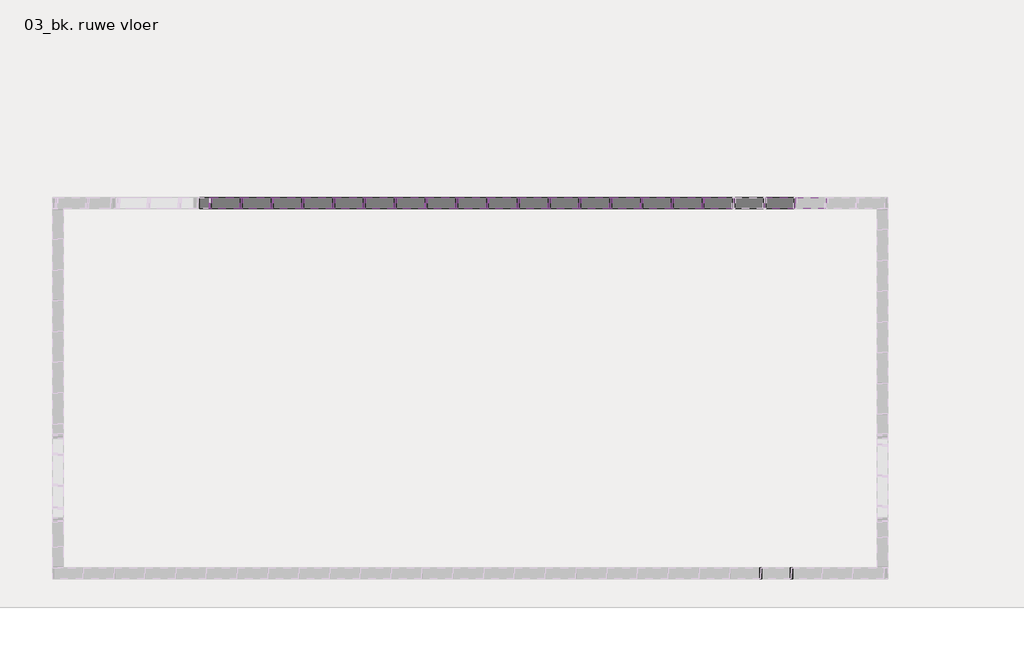
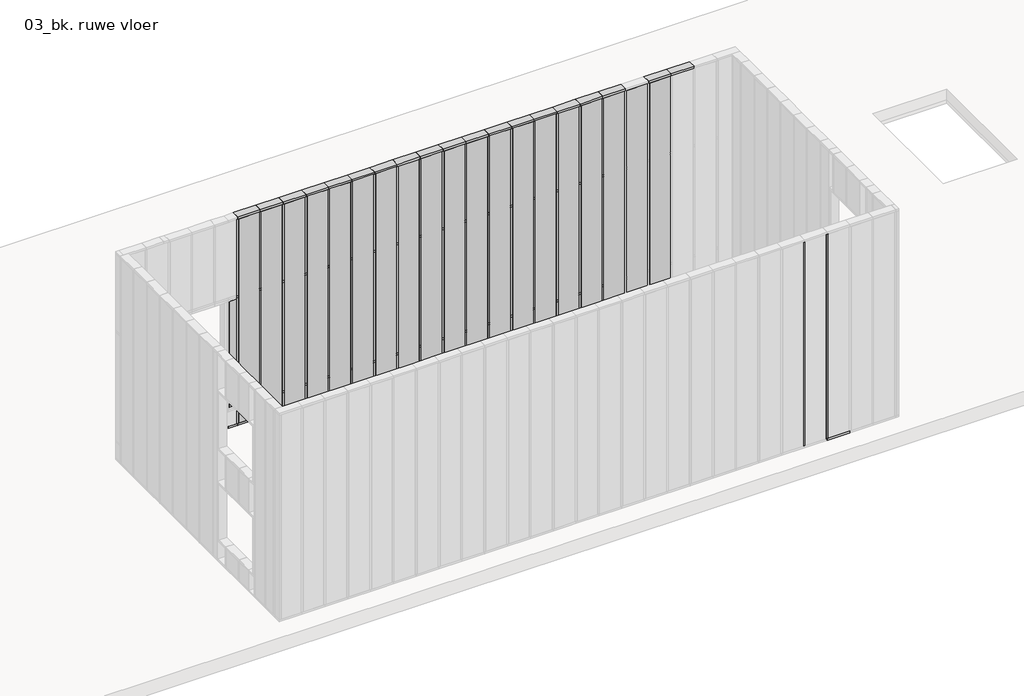
# One storey, part 3 of 9: 124 members, 20 plates.
"""IFC4 building model written with IfcOpenShell, lengths in millimetres."""

import ifcopenshell
import ifcopenshell.guid

model = None  # the IFC model being written
_history = None  # IfcOwnerHistory: only IFC2X3 demands one
_inside = {}  # id of a spatial element -> (the spatial element, [elements in it])
_under = {}  # id of a project, library or spatial element -> (it, [spatial elements below it])
_declared = {}  # id of a project -> (the project, [libraries it declares])
_typed = {}  # id of a type object -> (the type object, [elements of that type])
_made_of = {}  # id of a material, layer set ... -> (it, [elements and type objects made of it])


def new_model(schema):
    """Start an empty IFC model of exactly this schema.

    Asked for "IFC4X3", IfcOpenShell would pick the latest addendum, in which some entities
    have other attributes; the version numbers below select the first issue.
    IFC2X3 requires an IfcOwnerHistory on every rooted entity: one is made here for all.
    """
    global model, _history
    if schema == "IFC4X3":
        model = ifcopenshell.file(schema_version=(4, 3, 0, 0))
    else:
        model = ifcopenshell.file(schema=schema)
    _inside.clear()
    _under.clear()
    _declared.clear()
    _typed.clear()
    _made_of.clear()
    _history = None
    if model.schema == "IFC2X3":
        org = make("IfcOrganization", Name="unknown")
        user = make(
            "IfcPersonAndOrganization",
            ThePerson=make("IfcPerson", FamilyName="unknown"),
            TheOrganization=org,
        )
        app = make(
            "IfcApplication",
            ApplicationDeveloper=org,
            Version="unknown",
            ApplicationFullName="unknown",
            ApplicationIdentifier="unknown",
        )
        _history = make(
            "IfcOwnerHistory",
            OwningUser=user,
            OwningApplication=app,
            ChangeAction="ADDED",
            CreationDate=0,
        )
    return model


def make(cls, **values):
    """One entity of the class cls with the attributes given. An attribute that is None is left unset."""
    return model.create_entity(
        cls, **{name: value for name, value in values.items() if value is not None}
    )


def rooted(cls, **values):
    """An entity with a GlobalId (a new one), such as an element, a storey or a relation."""
    return make(cls, GlobalId=ifcopenshell.guid.new(), OwnerHistory=_history, **values)


def si_unit(unit_type, name, prefix=None):
    """IfcSIUnit, for example si_unit("LENGTHUNIT", "METRE", prefix="MILLI")."""
    return make("IfcSIUnit", UnitType=unit_type, Prefix=prefix, Name=name)


def assignment(units):
    """IfcUnitAssignment: the units of a project."""
    return None if units is None else make("IfcUnitAssignment", Units=units)


def point(xyz):
    """IfcCartesianPoint."""
    return None if xyz is None else make("IfcCartesianPoint", Coordinates=xyz)


def direction(xyz):
    """IfcDirection."""
    return None if xyz is None else make("IfcDirection", DirectionRatios=xyz)


def frame(location, z_axis=None, x_axis=None):
    """IfcAxis2Placement3D, a coordinate frame: its origin and axes. An axis left out is left unset."""
    return make(
        "IfcAxis2Placement3D",
        Location=point(location),
        Axis=direction(z_axis),
        RefDirection=direction(x_axis),
    )


def origin():
    """The frame at (0, 0, 0) with its axes left unset."""
    return frame((0.0, 0.0, 0.0))


def origin_with_axes():
    """The frame at (0, 0, 0) with the z axis (0, 0, 1) and the x axis (1, 0, 0) written out."""
    return frame((0.0, 0.0, 0.0), z_axis=(0.0, 0.0, 1.0), x_axis=(1.0, 0.0, 0.0))


def place(relative_to, where):
    """IfcLocalPlacement: puts the frame where relative to a parent placement (None: the world)."""
    return make(
        "IfcLocalPlacement", PlacementRelTo=relative_to, RelativePlacement=where
    )


def context(
    kind, dimensions, precision=None, world=None, true_north=None, identifier=None
):
    """IfcGeometricRepresentationContext, for example the 3D "Model" context."""
    return make(
        "IfcGeometricRepresentationContext",
        ContextIdentifier=identifier,
        ContextType=kind,
        CoordinateSpaceDimension=dimensions,
        Precision=precision,
        WorldCoordinateSystem=world,
        TrueNorth=true_north,
    )


def project(units=None, contexts=None):
    """IfcProject with its units and contexts."""
    return rooted(
        "IfcProject",
        Name="project",
        RepresentationContexts=contexts,
        UnitsInContext=assignment(units),
    )


def spatial(cls, under=None, at=None, **own):
    """A site, building, storey or space (cls), placed at a placement, below another one or the project."""
    s = rooted(cls, ObjectPlacement=at, **own)
    if under is not None:
        _under.setdefault(under.id(), (under, []))[1].append(s)
    return s


def polyline(points):
    """IfcPolyline through the points."""
    return make("IfcPolyline", Points=[point(p) for p in points])


def outline(outer, holes=None, kind="AREA"):
    """IfcArbitraryClosedProfileDef: a profile drawn as a closed curve; with holes, ...WithVoids."""
    if holes is None:
        return make("IfcArbitraryClosedProfileDef", ProfileType=kind, OuterCurve=outer)
    return make(
        "IfcArbitraryProfileDefWithVoids",
        ProfileType=kind,
        OuterCurve=outer,
        InnerCurves=holes,
    )


def extrude(swept, where, along, depth):
    """IfcExtrudedAreaSolid: the profile swept, set in the frame where, extruded along a direction by depth."""
    return make(
        "IfcExtrudedAreaSolid",
        SweptArea=swept,
        Position=where,
        ExtrudedDirection=direction(along),
        Depth=depth,
    )


def shape(context_of_items, identifier, shape_type, items):
    """IfcShapeRepresentation: the items that make up one representation, for example the "Body"."""
    return make(
        "IfcShapeRepresentation",
        ContextOfItems=context_of_items,
        RepresentationIdentifier=identifier,
        RepresentationType=shape_type,
        Items=items,
    )


def source(mapping_origin, context_of_items, identifier, shape_type, items):
    """IfcRepresentationMap: a shape defined once, which mapped items show again and again."""
    return make(
        "IfcRepresentationMap",
        MappingOrigin=mapping_origin,
        MappedRepresentation=shape(context_of_items, identifier, shape_type, items),
    )


def transform(
    local_origin,
    x_axis=None,
    y_axis=None,
    z_axis=None,
    scale=None,
    scale2=None,
    scale3=None,
    uniform=True,
):
    """IfcCartesianTransformationOperator3D, or its non-uniform kind. x_axis, y_axis, z_axis: its Axis1, 2, 3."""
    if uniform:
        return make(
            "IfcCartesianTransformationOperator3D",
            Axis1=direction(x_axis),
            Axis2=direction(y_axis),
            LocalOrigin=point(local_origin),
            Scale=scale,
            Axis3=direction(z_axis),
        )
    return make(
        "IfcCartesianTransformationOperator3DnonUniform",
        Axis1=direction(x_axis),
        Axis2=direction(y_axis),
        LocalOrigin=point(local_origin),
        Scale=scale,
        Axis3=direction(z_axis),
        Scale2=scale2,
        Scale3=scale3,
    )


def mapped(mapping_source, mapping_target):
    """IfcMappedItem: shows the shape of a source again, moved by a transform."""
    return make(
        "IfcMappedItem", MappingSource=mapping_source, MappingTarget=mapping_target
    )


def made_of(thing, what):
    """Note that an element or type object is made of a material, layer set ...; save() writes the relation."""
    if what is not None:
        _made_of.setdefault(what.id(), (what, []))[1].append(thing)
    return thing


def element(
    cls,
    number,
    at=None,
    inside=None,
    cuts=None,
    type_object=None,
    material=None,
    context=None,
    identifier="Body",
    shape_type=None,
    held_by="IfcProductDefinitionShape",
    body=None,
    shapes=None,
    **own,
):
    """One element of the class cls, such as IfcWall. Its Tag is "e" and its number.

    at: its placement. inside: the storey or other place that contains it. cuts: it is an
    opening in that element (IfcRelVoidsElement). A single representation is given by context,
    identifier, shape_type and body (its items); several are given by shapes. held_by: the class
    of the entity that holds the representations. save() writes the other relations.
    """
    e = rooted(cls, Tag="e%d" % number, ObjectPlacement=at, **own)
    if body is not None:
        shapes = [shape(context, identifier, shape_type, body)]
    if shapes is not None:
        e.Representation = make(held_by, Representations=shapes)
    if inside is not None:
        _inside.setdefault(inside.id(), (inside, []))[1].append(e)
    if cuts is not None:
        rooted(
            "IfcRelVoidsElement", RelatingBuildingElement=cuts, RelatedOpeningElement=e
        )
    if type_object is not None:
        _typed.setdefault(type_object.id(), (type_object, []))[1].append(e)
    return made_of(e, material)


def aggregate(whole, parts):
    """IfcRelAggregates: a whole, such as a stair, and the parts it consists of."""
    return rooted("IfcRelAggregates", RelatingObject=whole, RelatedObjects=parts)


def save(model, path):
    """Write the relations noted so far, then the file.

    IfcRelAggregates (storeys below a building ...), IfcRelContainedInSpatialStructure (elements
    in a storey), IfcRelDefinesByType, IfcRelAssociatesMaterial and IfcRelDeclares: one each for
    every whole, place, type object, material and project.
    """
    for whole, parts in _under.values():
        aggregate(whole, parts)
    for where, things in _inside.values():
        rooted(
            "IfcRelContainedInSpatialStructure",
            RelatedElements=things,
            RelatingStructure=where,
        )
    for kind, things in _typed.values():
        rooted("IfcRelDefinesByType", RelatedObjects=things, RelatingType=kind)
    for what, things in _made_of.values():
        rooted("IfcRelAssociatesMaterial", RelatedObjects=things, RelatingMaterial=what)
    for by, libraries in _declared.values():
        rooted("IfcRelDeclares", RelatingContext=by, RelatedDefinitions=libraries)
    model.write(path)


def rectangular_mullion_51268c3e(model_context):
    return source(origin(), model_context, "Body", "SweptSolid", [
        extrude(outline(polyline([(0.0, -71.0), (-38.0, -71.0), (-38.0, 71.0), (0.0, 71.0), (0.0, -71.0)])), frame((0.0, 0.0, -407.0), z_axis=(0.0, 0.0, 1.0), x_axis=(1.0, 0.0, 0.0)), (0.0, 0.0, 1.0), 407.0),
    ])


def rectangular_mullion_fd8aedfe(model_context):
    return source(origin(), model_context, "Body", "SweptSolid", [
        extrude(outline(polyline([(-38.0, -71.0), (-38.0, 71.0), (0.0, 71.0), (0.0, -71.0), (-38.0, -71.0)])), frame((0.0, 0.0, -407.0), z_axis=(0.0, 0.0, 1.0), x_axis=(1.0, 0.0, 0.0)), (0.0, 0.0, 1.0), 407.0),
    ])


def rectangular_mullion_bc699282(model_context):
    return source(origin(), model_context, "Body", "SweptSolid", [
        extrude(outline(polyline([(19.0, -71.0), (-19.0, -71.0), (-19.0, 71.0), (19.0, 71.0), (19.0, -71.0)])), frame((0.0, 0.0, -3849.0), z_axis=(0.0, 0.0, 1.0), x_axis=(1.0, 0.0, 0.0)), (0.0, 0.0, 1.0), 3849.0),
    ])


def rectangular_mullion_c53917db(model_context):
    return source(origin(), model_context, "Body", "SweptSolid", [
        extrude(outline(polyline([(19.0, -71.0), (-19.0, -71.0), (-19.0, 71.0), (19.0, 71.0), (19.0, -71.0)])), frame((0.0, 0.0, -295.0), z_axis=(0.0, 0.0, 1.0), x_axis=(1.0, 0.0, 0.0)), (0.0, 0.0, 1.0), 295.0),
    ])


def rectangular_mullion_c6f7c22d(model_context):
    return source(origin(), model_context, "Body", "SweptSolid", [
        extrude(outline(polyline([(-38.0, -71.0), (-38.0, 71.0), (0.0, 71.0), (0.0, -71.0), (-38.0, -71.0)])), frame((0.0, 0.0, -167.1558939), z_axis=(0.0, 0.0, 1.0), x_axis=(1.0, 0.0, 0.0)), (0.0, 0.0, 1.0), 167.1558939),
    ])


def rectangular_mullion_878a7b4c(model_context):
    return source(origin(), model_context, "Body", "SweptSolid", [
        extrude(outline(polyline([(19.0, -71.0), (-19.0, -71.0), (-19.0, 71.0), (19.0, 71.0), (19.0, -71.0)])), frame((0.0, 0.0, -1440.0), z_axis=(0.0, 0.0, 1.0), x_axis=(1.0, 0.0, 0.0)), (0.0, 0.0, 1.0), 1440.0),
    ])


def rectangular_mullion_c09c4bb1(model_context):
    return source(origin(), model_context, "Body", "SweptSolid", [
        extrude(outline(polyline([(19.0, -71.0), (-19.0, -71.0), (-19.0, 71.0), (19.0, 71.0), (19.0, -71.0)])), frame((0.0, 0.0, -38.0), z_axis=(0.0, 0.0, 1.0), x_axis=(1.0, 0.0, 0.0)), (0.0, 0.0, 1.0), 38.0),
    ])


def rectangular_mullion_39366410(model_context):
    return source(origin(), model_context, "Body", "SweptSolid", [
        extrude(outline(polyline([(19.0, -71.0), (-19.0, -71.0), (-19.0, 71.0), (19.0, 71.0), (19.0, -71.0)])), frame((0.0, 0.0, -2038.0), z_axis=(0.0, 0.0, 1.0), x_axis=(1.0, 0.0, 0.0)), (0.0, 0.0, 1.0), 2038.0),
    ])


def system_panel_efc5a8ab(model_context):
    return source(origin(), model_context, "Body", "SweptSolid", [
        extrude(outline(polyline([(0.0, -184.5), (0.0, 184.5), (295.0, 184.5), (333.0, 184.5), (2371.0, 184.5), (2409.0, 184.5), (3849.0, 184.5), (3849.0, -184.5), (2409.0, -184.5), (2371.0, -184.5), (333.0, -184.5), (295.0, -184.5), (0.0, -184.5)])), frame((0.0, -71.0, 0.0), z_axis=(0.0, 1.0, 0.0), x_axis=(0.0, 0.0, 1.0)), (0.0, 0.0, 1.0), 142.0),
    ])


def system_panel_6860f7c2(model_context):
    return source(origin(), model_context, "Body", "SweptSolid", [
        extrude(outline(polyline([(64.577947, -71.0), (-64.577947, -71.0), (-64.577947, 71.0), (64.577947, 71.0), (64.577947, -71.0)])), origin_with_axes(), (0.0, 0.0, 1.0), 2000.0),
    ])


model = new_model("IFC4")

# Units and contexts
model_context = context("Model", 3, world=origin())
ifc_project = project(units=[si_unit("LENGTHUNIT", "METRE", prefix="MILLI")], contexts=[model_context])

# Site, building, storey
site = spatial("IfcSite", under=ifc_project)
building = spatial("IfcBuilding", under=site)
storey = spatial("IfcBuildingStorey", under=building, Name="03_bk. ruwe vloer", Elevation=11330.0)

# Members
placement = place(None, origin())
rectangular_mullion_shape = rectangular_mullion_51268c3e(model_context)
element("IfcMember", 1, ObjectType="Rectangular Mullion", at=placement, inside=storey, context=model_context, shape_type="MappedRepresentation", body=[
    mapped(rectangular_mullion_shape, transform((63849.9999997, 5200.0, 15255.0), x_axis=(0.0, 0.0, 1.0), y_axis=(0.0, 1.0, 0.0), z_axis=(-1.0, 0.0, 0.0))),
])
element("IfcMember", 2, ObjectType="Rectangular Mullion", at=placement, inside=storey, context=model_context, shape_type="MappedRepresentation", body=[
    mapped(rectangular_mullion_shape, transform((63442.9999997, 5200.0, 15255.0), x_axis=(0.0, 0.0, 1.0), y_axis=(0.0, 1.0, 0.0), z_axis=(-1.0, 0.0, 0.0))),
])
element("IfcMember", 3, ObjectType="Rectangular Mullion", at=placement, inside=storey, context=model_context, shape_type="MappedRepresentation", body=[
    mapped(rectangular_mullion_shape, transform((62628.9999997, 5200.0, 15255.0), x_axis=(0.0, 0.0, 1.0), y_axis=(0.0, 1.0, 0.0), z_axis=(-1.0, 0.0, 0.0))),
])
element("IfcMember", 4, ObjectType="Rectangular Mullion", at=placement, inside=storey, context=model_context, shape_type="MappedRepresentation", body=[
    mapped(rectangular_mullion_shape, transform((62221.9999997, 5200.0, 15255.0), x_axis=(0.0, 0.0, 1.0), y_axis=(0.0, 1.0, 0.0), z_axis=(-1.0, 0.0, 0.0))),
])
element("IfcMember", 5, ObjectType="Rectangular Mullion", at=placement, inside=storey, context=model_context, shape_type="MappedRepresentation", body=[
    mapped(rectangular_mullion_shape, transform((61814.9999997, 5200.0, 15255.0), x_axis=(0.0, 0.0, 1.0), y_axis=(0.0, 1.0, 0.0), z_axis=(-1.0, 0.0, 0.0))),
])
element("IfcMember", 6, ObjectType="Rectangular Mullion", at=placement, inside=storey, context=model_context, shape_type="MappedRepresentation", body=[
    mapped(rectangular_mullion_shape, transform((61407.9999997, 5200.0, 15255.0), x_axis=(0.0, 0.0, 1.0), y_axis=(0.0, 1.0, 0.0), z_axis=(-1.0, 0.0, 0.0))),
])
element("IfcMember", 7, ObjectType="Rectangular Mullion", at=placement, inside=storey, context=model_context, shape_type="MappedRepresentation", body=[
    mapped(rectangular_mullion_shape, transform((61000.9999997, 5200.0, 15255.0), x_axis=(0.0, 0.0, 1.0), y_axis=(0.0, 1.0, 0.0), z_axis=(-1.0, 0.0, 0.0))),
])
element("IfcMember", 8, ObjectType="Rectangular Mullion", at=placement, inside=storey, context=model_context, shape_type="MappedRepresentation", body=[
    mapped(rectangular_mullion_shape, transform((60593.9999997, 5200.0, 15255.0), x_axis=(0.0, 0.0, 1.0), y_axis=(0.0, 1.0, 0.0), z_axis=(-1.0, 0.0, 0.0))),
])
element("IfcMember", 9, ObjectType="Rectangular Mullion", at=placement, inside=storey, context=model_context, shape_type="MappedRepresentation", body=[
    mapped(rectangular_mullion_shape, transform((60186.9999997, 5200.0, 15255.0), x_axis=(0.0, 0.0, 1.0), y_axis=(0.0, 1.0, 0.0), z_axis=(-1.0, 0.0, 0.0))),
])
element("IfcMember", 10, ObjectType="Rectangular Mullion", at=placement, inside=storey, context=model_context, shape_type="MappedRepresentation", body=[
    mapped(rectangular_mullion_shape, transform((59779.9999997, 5200.0, 15255.0), x_axis=(0.0, 0.0, 1.0), y_axis=(0.0, 1.0, 0.0), z_axis=(-1.0, 0.0, 0.0))),
])
element("IfcMember", 11, ObjectType="Rectangular Mullion", at=placement, inside=storey, context=model_context, shape_type="MappedRepresentation", body=[
    mapped(rectangular_mullion_shape, transform((59372.9999997, 5200.0, 15255.0), x_axis=(0.0, 0.0, 1.0), y_axis=(0.0, 1.0, 0.0), z_axis=(-1.0, 0.0, 0.0))),
])
element("IfcMember", 12, ObjectType="Rectangular Mullion", at=placement, inside=storey, context=model_context, shape_type="MappedRepresentation", body=[
    mapped(rectangular_mullion_shape, transform((58965.9999997, 5200.0, 15255.0), x_axis=(0.0, 0.0, 1.0), y_axis=(0.0, 1.0, 0.0), z_axis=(-1.0, 0.0, 0.0))),
])
element("IfcMember", 13, ObjectType="Rectangular Mullion", at=placement, inside=storey, context=model_context, shape_type="MappedRepresentation", body=[
    mapped(rectangular_mullion_shape, transform((58558.9999997, 5200.0, 15255.0), x_axis=(0.0, 0.0, 1.0), y_axis=(0.0, 1.0, 0.0), z_axis=(-1.0, 0.0, 0.0))),
])
element("IfcMember", 14, ObjectType="Rectangular Mullion", at=placement, inside=storey, context=model_context, shape_type="MappedRepresentation", body=[
    mapped(rectangular_mullion_shape, transform((58151.9999997, 5200.0, 15255.0), x_axis=(0.0, 0.0, 1.0), y_axis=(0.0, 1.0, 0.0), z_axis=(-1.0, 0.0, 0.0))),
])
element("IfcMember", 15, ObjectType="Rectangular Mullion", at=placement, inside=storey, context=model_context, shape_type="MappedRepresentation", body=[
    mapped(rectangular_mullion_shape, transform((57744.9999997, 5200.0, 15255.0), x_axis=(0.0, 0.0, 1.0), y_axis=(0.0, 1.0, 0.0), z_axis=(-1.0, 0.0, 0.0))),
])
element("IfcMember", 16, ObjectType="Rectangular Mullion", at=placement, inside=storey, context=model_context, shape_type="MappedRepresentation", body=[
    mapped(rectangular_mullion_shape, transform((57337.9999997, 5200.0, 15255.0), x_axis=(0.0, 0.0, 1.0), y_axis=(0.0, 1.0, 0.0), z_axis=(-1.0, 0.0, 0.0))),
])
element("IfcMember", 17, ObjectType="Rectangular Mullion", at=placement, inside=storey, context=model_context, shape_type="MappedRepresentation", body=[
    mapped(rectangular_mullion_shape, transform((56930.9999997, 5200.0, 15255.0), x_axis=(0.0, 0.0, 1.0), y_axis=(0.0, 1.0, 0.0), z_axis=(-1.0, 0.0, 0.0))),
])
element("IfcMember", 18, ObjectType="Rectangular Mullion", at=placement, inside=storey, context=model_context, shape_type="MappedRepresentation", body=[
    mapped(rectangular_mullion_shape, transform((56523.9999997, 5200.0, 15255.0), x_axis=(0.0, 0.0, 1.0), y_axis=(0.0, 1.0, 0.0), z_axis=(-1.0, 0.0, 0.0))),
])
element("IfcMember", 19, ObjectType="Rectangular Mullion", at=placement, inside=storey, context=model_context, shape_type="MappedRepresentation", body=[
    mapped(rectangular_mullion_shape, transform((56116.9999997, 5200.0, 15255.0), x_axis=(0.0, 0.0, 1.0), y_axis=(0.0, 1.0, 0.0), z_axis=(-1.0, 0.0, 0.0))),
])
rectangular_mullion_2_shape = rectangular_mullion_fd8aedfe(model_context)
element("IfcMember", 20, ObjectType="Rectangular Mullion", at=placement, inside=storey, context=model_context, shape_type="MappedRepresentation", body=[
    mapped(rectangular_mullion_2_shape, transform((62628.9999997, 5200.0, 11330.0), x_axis=(0.0, 0.0, -1.0), y_axis=(0.0, 1.0, 0.0), z_axis=(1.0, 0.0, 0.0))),
])
element("IfcMember", 21, ObjectType="Rectangular Mullion", at=placement, inside=storey, context=model_context, shape_type="MappedRepresentation", body=[
    mapped(rectangular_mullion_2_shape, transform((62221.9999997, 5200.0, 11330.0), x_axis=(0.0, 0.0, -1.0), y_axis=(0.0, 1.0, 0.0), z_axis=(1.0, 0.0, 0.0))),
])
element("IfcMember", 22, ObjectType="Rectangular Mullion", at=placement, inside=storey, context=model_context, shape_type="MappedRepresentation", body=[
    mapped(rectangular_mullion_2_shape, transform((61814.9999997, 5200.0, 11330.0), x_axis=(0.0, 0.0, -1.0), y_axis=(0.0, 1.0, 0.0), z_axis=(1.0, 0.0, 0.0))),
])
element("IfcMember", 23, ObjectType="Rectangular Mullion", at=placement, inside=storey, context=model_context, shape_type="MappedRepresentation", body=[
    mapped(rectangular_mullion_2_shape, transform((61407.9999997, 5200.0, 11330.0), x_axis=(0.0, 0.0, -1.0), y_axis=(0.0, 1.0, 0.0), z_axis=(1.0, 0.0, 0.0))),
])
element("IfcMember", 24, ObjectType="Rectangular Mullion", at=placement, inside=storey, context=model_context, shape_type="MappedRepresentation", body=[
    mapped(rectangular_mullion_2_shape, transform((61000.9999997, 5200.0, 11330.0), x_axis=(0.0, 0.0, -1.0), y_axis=(0.0, 1.0, 0.0), z_axis=(1.0, 0.0, 0.0))),
])
element("IfcMember", 25, ObjectType="Rectangular Mullion", at=placement, inside=storey, context=model_context, shape_type="MappedRepresentation", body=[
    mapped(rectangular_mullion_2_shape, transform((60593.9999997, 5200.0, 11330.0), x_axis=(0.0, 0.0, -1.0), y_axis=(0.0, 1.0, 0.0), z_axis=(1.0, 0.0, 0.0))),
])
element("IfcMember", 26, ObjectType="Rectangular Mullion", at=placement, inside=storey, context=model_context, shape_type="MappedRepresentation", body=[
    mapped(rectangular_mullion_2_shape, transform((60186.9999997, 5200.0, 11330.0), x_axis=(0.0, 0.0, -1.0), y_axis=(0.0, 1.0, 0.0), z_axis=(1.0, 0.0, 0.0))),
])
element("IfcMember", 27, ObjectType="Rectangular Mullion", at=placement, inside=storey, context=model_context, shape_type="MappedRepresentation", body=[
    mapped(rectangular_mullion_2_shape, transform((59779.9999997, 5200.0, 11330.0), x_axis=(0.0, 0.0, -1.0), y_axis=(0.0, 1.0, 0.0), z_axis=(1.0, 0.0, 0.0))),
])
element("IfcMember", 28, ObjectType="Rectangular Mullion", at=placement, inside=storey, context=model_context, shape_type="MappedRepresentation", body=[
    mapped(rectangular_mullion_2_shape, transform((59372.9999997, 5200.0, 11330.0), x_axis=(0.0, 0.0, -1.0), y_axis=(0.0, 1.0, 0.0), z_axis=(1.0, 0.0, 0.0))),
])
element("IfcMember", 29, ObjectType="Rectangular Mullion", at=placement, inside=storey, context=model_context, shape_type="MappedRepresentation", body=[
    mapped(rectangular_mullion_2_shape, transform((58965.9999997, 5200.0, 11330.0), x_axis=(0.0, 0.0, -1.0), y_axis=(0.0, 1.0, 0.0), z_axis=(1.0, 0.0, 0.0))),
])
element("IfcMember", 30, ObjectType="Rectangular Mullion", at=placement, inside=storey, context=model_context, shape_type="MappedRepresentation", body=[
    mapped(rectangular_mullion_2_shape, transform((58558.9999997, 5200.0, 11330.0), x_axis=(0.0, 0.0, -1.0), y_axis=(0.0, 1.0, 0.0), z_axis=(1.0, 0.0, 0.0))),
])
element("IfcMember", 31, ObjectType="Rectangular Mullion", at=placement, inside=storey, context=model_context, shape_type="MappedRepresentation", body=[
    mapped(rectangular_mullion_2_shape, transform((58151.9999997, 5200.0, 11330.0), x_axis=(0.0, 0.0, -1.0), y_axis=(0.0, 1.0, 0.0), z_axis=(1.0, 0.0, 0.0))),
])
element("IfcMember", 32, ObjectType="Rectangular Mullion", at=placement, inside=storey, context=model_context, shape_type="MappedRepresentation", body=[
    mapped(rectangular_mullion_2_shape, transform((57744.9999997, 5200.0, 11330.0), x_axis=(0.0, 0.0, -1.0), y_axis=(0.0, 1.0, 0.0), z_axis=(1.0, 0.0, 0.0))),
])
element("IfcMember", 33, ObjectType="Rectangular Mullion", at=placement, inside=storey, context=model_context, shape_type="MappedRepresentation", body=[
    mapped(rectangular_mullion_2_shape, transform((57337.9999997, 5200.0, 11330.0), x_axis=(0.0, 0.0, -1.0), y_axis=(0.0, 1.0, 0.0), z_axis=(1.0, 0.0, 0.0))),
])
element("IfcMember", 34, ObjectType="Rectangular Mullion", at=placement, inside=storey, context=model_context, shape_type="MappedRepresentation", body=[
    mapped(rectangular_mullion_2_shape, transform((56930.9999997, 5200.0, 11330.0), x_axis=(0.0, 0.0, -1.0), y_axis=(0.0, 1.0, 0.0), z_axis=(1.0, 0.0, 0.0))),
])
element("IfcMember", 35, ObjectType="Rectangular Mullion", at=placement, inside=storey, context=model_context, shape_type="MappedRepresentation", body=[
    mapped(rectangular_mullion_2_shape, transform((63797.0000003, 300.0, 11330.0), x_axis=(0.0, 0.0, -1.0), y_axis=(0.0, -1.0, 0.0), z_axis=(-1.0, 0.0, 0.0))),
])
element("IfcMember", 36, ObjectType="Rectangular Mullion", at=placement, inside=storey, context=model_context, shape_type="MappedRepresentation", body=[
    mapped(rectangular_mullion_2_shape, transform((56523.9999997, 5200.0, 11330.0), x_axis=(0.0, 0.0, -1.0), y_axis=(0.0, 1.0, 0.0), z_axis=(1.0, 0.0, 0.0))),
])
rectangular_mullion_3_shape = rectangular_mullion_bc699282(model_context)
element("IfcMember", 37, ObjectType="Rectangular Mullion", at=placement, inside=storey, context=model_context, shape_type="MappedRepresentation", body=[
    mapped(rectangular_mullion_3_shape, transform((63390.0000003, 300.0, 11368.0), x_axis=(1.0, 0.0, 0.0), y_axis=(0.0, -1.0, 0.0), z_axis=(0.0, 0.0, -1.0))),
])
element("IfcMember", 38, ObjectType="Rectangular Mullion", at=placement, inside=storey, context=model_context, shape_type="MappedRepresentation", body=[
    mapped(rectangular_mullion_3_shape, transform((63797.0000003, 300.0, 11368.0), x_axis=(1.0, 0.0, 0.0), y_axis=(0.0, -1.0, 0.0), z_axis=(0.0, 0.0, -1.0))),
])
rectangular_mullion_4_shape = rectangular_mullion_c53917db(model_context)
element("IfcMember", 39, ObjectType="Rectangular Mullion", at=placement, inside=storey, context=model_context, shape_type="MappedRepresentation", body=[
    mapped(rectangular_mullion_4_shape, transform((62628.9999997, 5200.0, 11368.0), x_axis=(-1.0, 0.0, 0.0), y_axis=(0.0, 1.0, 0.0), z_axis=(0.0, 0.0, -1.0))),
])
element("IfcMember", 40, ObjectType="Rectangular Mullion", at=placement, inside=storey, context=model_context, shape_type="MappedRepresentation", body=[
    mapped(rectangular_mullion_4_shape, transform((62221.9999997, 5200.0, 11368.0), x_axis=(-1.0, 0.0, 0.0), y_axis=(0.0, 1.0, 0.0), z_axis=(0.0, 0.0, -1.0))),
])
element("IfcMember", 41, ObjectType="Rectangular Mullion", at=placement, inside=storey, context=model_context, shape_type="MappedRepresentation", body=[
    mapped(rectangular_mullion_4_shape, transform((61814.9999997, 5200.0, 11368.0), x_axis=(-1.0, 0.0, 0.0), y_axis=(0.0, 1.0, 0.0), z_axis=(0.0, 0.0, -1.0))),
])
element("IfcMember", 42, ObjectType="Rectangular Mullion", at=placement, inside=storey, context=model_context, shape_type="MappedRepresentation", body=[
    mapped(rectangular_mullion_4_shape, transform((61407.9999997, 5200.0, 11368.0), x_axis=(-1.0, 0.0, 0.0), y_axis=(0.0, 1.0, 0.0), z_axis=(0.0, 0.0, -1.0))),
])
element("IfcMember", 43, ObjectType="Rectangular Mullion", at=placement, inside=storey, context=model_context, shape_type="MappedRepresentation", body=[
    mapped(rectangular_mullion_4_shape, transform((61000.9999997, 5200.0, 11368.0), x_axis=(-1.0, 0.0, 0.0), y_axis=(0.0, 1.0, 0.0), z_axis=(0.0, 0.0, -1.0))),
])
element("IfcMember", 44, ObjectType="Rectangular Mullion", at=placement, inside=storey, context=model_context, shape_type="MappedRepresentation", body=[
    mapped(rectangular_mullion_4_shape, transform((60593.9999997, 5200.0, 11368.0), x_axis=(-1.0, 0.0, 0.0), y_axis=(0.0, 1.0, 0.0), z_axis=(0.0, 0.0, -1.0))),
])
element("IfcMember", 45, ObjectType="Rectangular Mullion", at=placement, inside=storey, context=model_context, shape_type="MappedRepresentation", body=[
    mapped(rectangular_mullion_4_shape, transform((60186.9999997, 5200.0, 11368.0), x_axis=(-1.0, 0.0, 0.0), y_axis=(0.0, 1.0, 0.0), z_axis=(0.0, 0.0, -1.0))),
])
element("IfcMember", 46, ObjectType="Rectangular Mullion", at=placement, inside=storey, context=model_context, shape_type="MappedRepresentation", body=[
    mapped(rectangular_mullion_4_shape, transform((59779.9999997, 5200.0, 11368.0), x_axis=(-1.0, 0.0, 0.0), y_axis=(0.0, 1.0, 0.0), z_axis=(0.0, 0.0, -1.0))),
])
element("IfcMember", 47, ObjectType="Rectangular Mullion", at=placement, inside=storey, context=model_context, shape_type="MappedRepresentation", body=[
    mapped(rectangular_mullion_4_shape, transform((59372.9999997, 5200.0, 11368.0), x_axis=(-1.0, 0.0, 0.0), y_axis=(0.0, 1.0, 0.0), z_axis=(0.0, 0.0, -1.0))),
])
element("IfcMember", 48, ObjectType="Rectangular Mullion", at=placement, inside=storey, context=model_context, shape_type="MappedRepresentation", body=[
    mapped(rectangular_mullion_4_shape, transform((58965.9999997, 5200.0, 11368.0), x_axis=(-1.0, 0.0, 0.0), y_axis=(0.0, 1.0, 0.0), z_axis=(0.0, 0.0, -1.0))),
])
element("IfcMember", 49, ObjectType="Rectangular Mullion", at=placement, inside=storey, context=model_context, shape_type="MappedRepresentation", body=[
    mapped(rectangular_mullion_4_shape, transform((58558.9999997, 5200.0, 11368.0), x_axis=(-1.0, 0.0, 0.0), y_axis=(0.0, 1.0, 0.0), z_axis=(0.0, 0.0, -1.0))),
])
element("IfcMember", 50, ObjectType="Rectangular Mullion", at=placement, inside=storey, context=model_context, shape_type="MappedRepresentation", body=[
    mapped(rectangular_mullion_4_shape, transform((58151.9999997, 5200.0, 11368.0), x_axis=(-1.0, 0.0, 0.0), y_axis=(0.0, 1.0, 0.0), z_axis=(0.0, 0.0, -1.0))),
])
element("IfcMember", 51, ObjectType="Rectangular Mullion", at=placement, inside=storey, context=model_context, shape_type="MappedRepresentation", body=[
    mapped(rectangular_mullion_4_shape, transform((57744.9999997, 5200.0, 11368.0), x_axis=(-1.0, 0.0, 0.0), y_axis=(0.0, 1.0, 0.0), z_axis=(0.0, 0.0, -1.0))),
])
element("IfcMember", 52, ObjectType="Rectangular Mullion", at=placement, inside=storey, context=model_context, shape_type="MappedRepresentation", body=[
    mapped(rectangular_mullion_4_shape, transform((57337.9999997, 5200.0, 11368.0), x_axis=(-1.0, 0.0, 0.0), y_axis=(0.0, 1.0, 0.0), z_axis=(0.0, 0.0, -1.0))),
])
element("IfcMember", 53, ObjectType="Rectangular Mullion", at=placement, inside=storey, context=model_context, shape_type="MappedRepresentation", body=[
    mapped(rectangular_mullion_4_shape, transform((56930.9999997, 5200.0, 11368.0), x_axis=(-1.0, 0.0, 0.0), y_axis=(0.0, 1.0, 0.0), z_axis=(0.0, 0.0, -1.0))),
])
element("IfcMember", 54, ObjectType="Rectangular Mullion", at=placement, inside=storey, context=model_context, shape_type="MappedRepresentation", body=[
    mapped(rectangular_mullion_4_shape, transform((56523.9999997, 5200.0, 11368.0), x_axis=(-1.0, 0.0, 0.0), y_axis=(0.0, 1.0, 0.0), z_axis=(0.0, 0.0, -1.0))),
])
element("IfcMember", 55, ObjectType="Rectangular Mullion", at=placement, inside=storey, context=model_context, shape_type="MappedRepresentation", body=[
    mapped(rectangular_mullion_4_shape, transform((56116.9999997, 5200.0, 11368.0), x_axis=(-1.0, 0.0, 0.0), y_axis=(0.0, 1.0, 0.0), z_axis=(0.0, 0.0, -1.0))),
])
rectangular_mullion_5_shape = rectangular_mullion_c6f7c22d(model_context)
element("IfcMember", 56, ObjectType="Rectangular Mullion", at=placement, inside=storey, context=model_context, shape_type="MappedRepresentation", body=[
    mapped(rectangular_mullion_5_shape, transform((56116.9999997, 5200.0, 11330.0), x_axis=(0.0, 0.0, -1.0), y_axis=(0.0, 1.0, 0.0), z_axis=(1.0, 0.0, 0.0))),
])
rectangular_mullion_6_shape = rectangular_mullion_878a7b4c(model_context)
element("IfcMember", 57, ObjectType="Rectangular Mullion", at=placement, inside=storey, context=model_context, shape_type="MappedRepresentation", body=[
    mapped(rectangular_mullion_6_shape, transform((62628.9999997, 5200.0, 13777.0), x_axis=(-1.0, 0.0, 0.0), y_axis=(0.0, 1.0, 0.0), z_axis=(0.0, 0.0, -1.0))),
])
element("IfcMember", 58, ObjectType="Rectangular Mullion", at=placement, inside=storey, context=model_context, shape_type="MappedRepresentation", body=[
    mapped(rectangular_mullion_6_shape, transform((62221.9999997, 5200.0, 13777.0), x_axis=(-1.0, 0.0, 0.0), y_axis=(0.0, 1.0, 0.0), z_axis=(0.0, 0.0, -1.0))),
])
element("IfcMember", 59, ObjectType="Rectangular Mullion", at=placement, inside=storey, context=model_context, shape_type="MappedRepresentation", body=[
    mapped(rectangular_mullion_6_shape, transform((61814.9999997, 5200.0, 13777.0), x_axis=(-1.0, 0.0, 0.0), y_axis=(0.0, 1.0, 0.0), z_axis=(0.0, 0.0, -1.0))),
])
element("IfcMember", 60, ObjectType="Rectangular Mullion", at=placement, inside=storey, context=model_context, shape_type="MappedRepresentation", body=[
    mapped(rectangular_mullion_6_shape, transform((61407.9999997, 5200.0, 13777.0), x_axis=(-1.0, 0.0, 0.0), y_axis=(0.0, 1.0, 0.0), z_axis=(0.0, 0.0, -1.0))),
])
element("IfcMember", 61, ObjectType="Rectangular Mullion", at=placement, inside=storey, context=model_context, shape_type="MappedRepresentation", body=[
    mapped(rectangular_mullion_6_shape, transform((61000.9999997, 5200.0, 13777.0), x_axis=(-1.0, 0.0, 0.0), y_axis=(0.0, 1.0, 0.0), z_axis=(0.0, 0.0, -1.0))),
])
element("IfcMember", 62, ObjectType="Rectangular Mullion", at=placement, inside=storey, context=model_context, shape_type="MappedRepresentation", body=[
    mapped(rectangular_mullion_6_shape, transform((60593.9999997, 5200.0, 13777.0), x_axis=(-1.0, 0.0, 0.0), y_axis=(0.0, 1.0, 0.0), z_axis=(0.0, 0.0, -1.0))),
])
element("IfcMember", 63, ObjectType="Rectangular Mullion", at=placement, inside=storey, context=model_context, shape_type="MappedRepresentation", body=[
    mapped(rectangular_mullion_6_shape, transform((60186.9999997, 5200.0, 13777.0), x_axis=(-1.0, 0.0, 0.0), y_axis=(0.0, 1.0, 0.0), z_axis=(0.0, 0.0, -1.0))),
])
element("IfcMember", 64, ObjectType="Rectangular Mullion", at=placement, inside=storey, context=model_context, shape_type="MappedRepresentation", body=[
    mapped(rectangular_mullion_6_shape, transform((59779.9999997, 5200.0, 13777.0), x_axis=(-1.0, 0.0, 0.0), y_axis=(0.0, 1.0, 0.0), z_axis=(0.0, 0.0, -1.0))),
])
element("IfcMember", 65, ObjectType="Rectangular Mullion", at=placement, inside=storey, context=model_context, shape_type="MappedRepresentation", body=[
    mapped(rectangular_mullion_6_shape, transform((59372.9999997, 5200.0, 13777.0), x_axis=(-1.0, 0.0, 0.0), y_axis=(0.0, 1.0, 0.0), z_axis=(0.0, 0.0, -1.0))),
])
element("IfcMember", 66, ObjectType="Rectangular Mullion", at=placement, inside=storey, context=model_context, shape_type="MappedRepresentation", body=[
    mapped(rectangular_mullion_6_shape, transform((58965.9999997, 5200.0, 13777.0), x_axis=(-1.0, 0.0, 0.0), y_axis=(0.0, 1.0, 0.0), z_axis=(0.0, 0.0, -1.0))),
])
element("IfcMember", 67, ObjectType="Rectangular Mullion", at=placement, inside=storey, context=model_context, shape_type="MappedRepresentation", body=[
    mapped(rectangular_mullion_6_shape, transform((58558.9999997, 5200.0, 13777.0), x_axis=(-1.0, 0.0, 0.0), y_axis=(0.0, 1.0, 0.0), z_axis=(0.0, 0.0, -1.0))),
])
element("IfcMember", 68, ObjectType="Rectangular Mullion", at=placement, inside=storey, context=model_context, shape_type="MappedRepresentation", body=[
    mapped(rectangular_mullion_6_shape, transform((58151.9999997, 5200.0, 13777.0), x_axis=(-1.0, 0.0, 0.0), y_axis=(0.0, 1.0, 0.0), z_axis=(0.0, 0.0, -1.0))),
])
element("IfcMember", 69, ObjectType="Rectangular Mullion", at=placement, inside=storey, context=model_context, shape_type="MappedRepresentation", body=[
    mapped(rectangular_mullion_6_shape, transform((57744.9999997, 5200.0, 13777.0), x_axis=(-1.0, 0.0, 0.0), y_axis=(0.0, 1.0, 0.0), z_axis=(0.0, 0.0, -1.0))),
])
element("IfcMember", 70, ObjectType="Rectangular Mullion", at=placement, inside=storey, context=model_context, shape_type="MappedRepresentation", body=[
    mapped(rectangular_mullion_6_shape, transform((57337.9999997, 5200.0, 13777.0), x_axis=(-1.0, 0.0, 0.0), y_axis=(0.0, 1.0, 0.0), z_axis=(0.0, 0.0, -1.0))),
])
element("IfcMember", 71, ObjectType="Rectangular Mullion", at=placement, inside=storey, context=model_context, shape_type="MappedRepresentation", body=[
    mapped(rectangular_mullion_6_shape, transform((56930.9999997, 5200.0, 13777.0), x_axis=(-1.0, 0.0, 0.0), y_axis=(0.0, 1.0, 0.0), z_axis=(0.0, 0.0, -1.0))),
])
element("IfcMember", 72, ObjectType="Rectangular Mullion", at=placement, inside=storey, context=model_context, shape_type="MappedRepresentation", body=[
    mapped(rectangular_mullion_6_shape, transform((56523.9999997, 5200.0, 13777.0), x_axis=(-1.0, 0.0, 0.0), y_axis=(0.0, 1.0, 0.0), z_axis=(0.0, 0.0, -1.0))),
])
element("IfcMember", 73, ObjectType="Rectangular Mullion", at=placement, inside=storey, context=model_context, shape_type="MappedRepresentation", body=[
    mapped(rectangular_mullion_6_shape, transform((56116.9999997, 5200.0, 13777.0), x_axis=(-1.0, 0.0, 0.0), y_axis=(0.0, 1.0, 0.0), z_axis=(0.0, 0.0, -1.0))),
])
rectangular_mullion_7_shape = rectangular_mullion_c09c4bb1(model_context)
element("IfcMember", 74, ObjectType="Rectangular Mullion", at=placement, inside=storey, context=model_context, shape_type="MappedRepresentation", body=[
    mapped(rectangular_mullion_7_shape, transform((62628.9999997, 5200.0, 13739.0), x_axis=(-1.0, 0.0, 0.0), y_axis=(0.0, 1.0, 0.0), z_axis=(0.0, 0.0, -1.0))),
])
element("IfcMember", 75, ObjectType="Rectangular Mullion", at=placement, inside=storey, context=model_context, shape_type="MappedRepresentation", body=[
    mapped(rectangular_mullion_7_shape, transform((62221.9999997, 5200.0, 13739.0), x_axis=(-1.0, 0.0, 0.0), y_axis=(0.0, 1.0, 0.0), z_axis=(0.0, 0.0, -1.0))),
])
element("IfcMember", 76, ObjectType="Rectangular Mullion", at=placement, inside=storey, context=model_context, shape_type="MappedRepresentation", body=[
    mapped(rectangular_mullion_7_shape, transform((61814.9999997, 5200.0, 13739.0), x_axis=(-1.0, 0.0, 0.0), y_axis=(0.0, 1.0, 0.0), z_axis=(0.0, 0.0, -1.0))),
])
element("IfcMember", 77, ObjectType="Rectangular Mullion", at=placement, inside=storey, context=model_context, shape_type="MappedRepresentation", body=[
    mapped(rectangular_mullion_7_shape, transform((61407.9999997, 5200.0, 13739.0), x_axis=(-1.0, 0.0, 0.0), y_axis=(0.0, 1.0, 0.0), z_axis=(0.0, 0.0, -1.0))),
])
element("IfcMember", 78, ObjectType="Rectangular Mullion", at=placement, inside=storey, context=model_context, shape_type="MappedRepresentation", body=[
    mapped(rectangular_mullion_7_shape, transform((61000.9999997, 5200.0, 13739.0), x_axis=(-1.0, 0.0, 0.0), y_axis=(0.0, 1.0, 0.0), z_axis=(0.0, 0.0, -1.0))),
])
element("IfcMember", 79, ObjectType="Rectangular Mullion", at=placement, inside=storey, context=model_context, shape_type="MappedRepresentation", body=[
    mapped(rectangular_mullion_7_shape, transform((60593.9999997, 5200.0, 13739.0), x_axis=(-1.0, 0.0, 0.0), y_axis=(0.0, 1.0, 0.0), z_axis=(0.0, 0.0, -1.0))),
])
element("IfcMember", 80, ObjectType="Rectangular Mullion", at=placement, inside=storey, context=model_context, shape_type="MappedRepresentation", body=[
    mapped(rectangular_mullion_7_shape, transform((60186.9999997, 5200.0, 13739.0), x_axis=(-1.0, 0.0, 0.0), y_axis=(0.0, 1.0, 0.0), z_axis=(0.0, 0.0, -1.0))),
])
element("IfcMember", 81, ObjectType="Rectangular Mullion", at=placement, inside=storey, context=model_context, shape_type="MappedRepresentation", body=[
    mapped(rectangular_mullion_7_shape, transform((59779.9999997, 5200.0, 13739.0), x_axis=(-1.0, 0.0, 0.0), y_axis=(0.0, 1.0, 0.0), z_axis=(0.0, 0.0, -1.0))),
])
element("IfcMember", 82, ObjectType="Rectangular Mullion", at=placement, inside=storey, context=model_context, shape_type="MappedRepresentation", body=[
    mapped(rectangular_mullion_7_shape, transform((59372.9999997, 5200.0, 13739.0), x_axis=(-1.0, 0.0, 0.0), y_axis=(0.0, 1.0, 0.0), z_axis=(0.0, 0.0, -1.0))),
])
element("IfcMember", 83, ObjectType="Rectangular Mullion", at=placement, inside=storey, context=model_context, shape_type="MappedRepresentation", body=[
    mapped(rectangular_mullion_7_shape, transform((58965.9999997, 5200.0, 13739.0), x_axis=(-1.0, 0.0, 0.0), y_axis=(0.0, 1.0, 0.0), z_axis=(0.0, 0.0, -1.0))),
])
element("IfcMember", 84, ObjectType="Rectangular Mullion", at=placement, inside=storey, context=model_context, shape_type="MappedRepresentation", body=[
    mapped(rectangular_mullion_7_shape, transform((58558.9999997, 5200.0, 13739.0), x_axis=(-1.0, 0.0, 0.0), y_axis=(0.0, 1.0, 0.0), z_axis=(0.0, 0.0, -1.0))),
])
element("IfcMember", 85, ObjectType="Rectangular Mullion", at=placement, inside=storey, context=model_context, shape_type="MappedRepresentation", body=[
    mapped(rectangular_mullion_7_shape, transform((58151.9999997, 5200.0, 13739.0), x_axis=(-1.0, 0.0, 0.0), y_axis=(0.0, 1.0, 0.0), z_axis=(0.0, 0.0, -1.0))),
])
element("IfcMember", 86, ObjectType="Rectangular Mullion", at=placement, inside=storey, context=model_context, shape_type="MappedRepresentation", body=[
    mapped(rectangular_mullion_7_shape, transform((57744.9999997, 5200.0, 13739.0), x_axis=(-1.0, 0.0, 0.0), y_axis=(0.0, 1.0, 0.0), z_axis=(0.0, 0.0, -1.0))),
])
element("IfcMember", 87, ObjectType="Rectangular Mullion", at=placement, inside=storey, context=model_context, shape_type="MappedRepresentation", body=[
    mapped(rectangular_mullion_7_shape, transform((57337.9999997, 5200.0, 13739.0), x_axis=(-1.0, 0.0, 0.0), y_axis=(0.0, 1.0, 0.0), z_axis=(0.0, 0.0, -1.0))),
])
element("IfcMember", 88, ObjectType="Rectangular Mullion", at=placement, inside=storey, context=model_context, shape_type="MappedRepresentation", body=[
    mapped(rectangular_mullion_7_shape, transform((56930.9999997, 5200.0, 13739.0), x_axis=(-1.0, 0.0, 0.0), y_axis=(0.0, 1.0, 0.0), z_axis=(0.0, 0.0, -1.0))),
])
element("IfcMember", 89, ObjectType="Rectangular Mullion", at=placement, inside=storey, context=model_context, shape_type="MappedRepresentation", body=[
    mapped(rectangular_mullion_7_shape, transform((56523.9999997, 5200.0, 13739.0), x_axis=(-1.0, 0.0, 0.0), y_axis=(0.0, 1.0, 0.0), z_axis=(0.0, 0.0, -1.0))),
])
element("IfcMember", 90, ObjectType="Rectangular Mullion", at=placement, inside=storey, context=model_context, shape_type="MappedRepresentation", body=[
    mapped(rectangular_mullion_7_shape, transform((62628.9999997, 5200.0, 11663.0), x_axis=(-1.0, 0.0, 0.0), y_axis=(0.0, 1.0, 0.0), z_axis=(0.0, 0.0, -1.0))),
])
element("IfcMember", 91, ObjectType="Rectangular Mullion", at=placement, inside=storey, context=model_context, shape_type="MappedRepresentation", body=[
    mapped(rectangular_mullion_7_shape, transform((62221.9999997, 5200.0, 11663.0), x_axis=(-1.0, 0.0, 0.0), y_axis=(0.0, 1.0, 0.0), z_axis=(0.0, 0.0, -1.0))),
])
element("IfcMember", 92, ObjectType="Rectangular Mullion", at=placement, inside=storey, context=model_context, shape_type="MappedRepresentation", body=[
    mapped(rectangular_mullion_7_shape, transform((61814.9999997, 5200.0, 11663.0), x_axis=(-1.0, 0.0, 0.0), y_axis=(0.0, 1.0, 0.0), z_axis=(0.0, 0.0, -1.0))),
])
element("IfcMember", 93, ObjectType="Rectangular Mullion", at=placement, inside=storey, context=model_context, shape_type="MappedRepresentation", body=[
    mapped(rectangular_mullion_7_shape, transform((61407.9999997, 5200.0, 11663.0), x_axis=(-1.0, 0.0, 0.0), y_axis=(0.0, 1.0, 0.0), z_axis=(0.0, 0.0, -1.0))),
])
element("IfcMember", 94, ObjectType="Rectangular Mullion", at=placement, inside=storey, context=model_context, shape_type="MappedRepresentation", body=[
    mapped(rectangular_mullion_7_shape, transform((61000.9999997, 5200.0, 11663.0), x_axis=(-1.0, 0.0, 0.0), y_axis=(0.0, 1.0, 0.0), z_axis=(0.0, 0.0, -1.0))),
])
element("IfcMember", 95, ObjectType="Rectangular Mullion", at=placement, inside=storey, context=model_context, shape_type="MappedRepresentation", body=[
    mapped(rectangular_mullion_7_shape, transform((60593.9999997, 5200.0, 11663.0), x_axis=(-1.0, 0.0, 0.0), y_axis=(0.0, 1.0, 0.0), z_axis=(0.0, 0.0, -1.0))),
])
element("IfcMember", 96, ObjectType="Rectangular Mullion", at=placement, inside=storey, context=model_context, shape_type="MappedRepresentation", body=[
    mapped(rectangular_mullion_7_shape, transform((60186.9999997, 5200.0, 11663.0), x_axis=(-1.0, 0.0, 0.0), y_axis=(0.0, 1.0, 0.0), z_axis=(0.0, 0.0, -1.0))),
])
element("IfcMember", 97, ObjectType="Rectangular Mullion", at=placement, inside=storey, context=model_context, shape_type="MappedRepresentation", body=[
    mapped(rectangular_mullion_7_shape, transform((59779.9999997, 5200.0, 11663.0), x_axis=(-1.0, 0.0, 0.0), y_axis=(0.0, 1.0, 0.0), z_axis=(0.0, 0.0, -1.0))),
])
element("IfcMember", 98, ObjectType="Rectangular Mullion", at=placement, inside=storey, context=model_context, shape_type="MappedRepresentation", body=[
    mapped(rectangular_mullion_7_shape, transform((59372.9999997, 5200.0, 11663.0), x_axis=(-1.0, 0.0, 0.0), y_axis=(0.0, 1.0, 0.0), z_axis=(0.0, 0.0, -1.0))),
])
element("IfcMember", 99, ObjectType="Rectangular Mullion", at=placement, inside=storey, context=model_context, shape_type="MappedRepresentation", body=[
    mapped(rectangular_mullion_7_shape, transform((58965.9999997, 5200.0, 11663.0), x_axis=(-1.0, 0.0, 0.0), y_axis=(0.0, 1.0, 0.0), z_axis=(0.0, 0.0, -1.0))),
])
element("IfcMember", 100, ObjectType="Rectangular Mullion", at=placement, inside=storey, context=model_context, shape_type="MappedRepresentation", body=[
    mapped(rectangular_mullion_7_shape, transform((58558.9999997, 5200.0, 11663.0), x_axis=(-1.0, 0.0, 0.0), y_axis=(0.0, 1.0, 0.0), z_axis=(0.0, 0.0, -1.0))),
])
element("IfcMember", 101, ObjectType="Rectangular Mullion", at=placement, inside=storey, context=model_context, shape_type="MappedRepresentation", body=[
    mapped(rectangular_mullion_7_shape, transform((58151.9999997, 5200.0, 11663.0), x_axis=(-1.0, 0.0, 0.0), y_axis=(0.0, 1.0, 0.0), z_axis=(0.0, 0.0, -1.0))),
])
element("IfcMember", 102, ObjectType="Rectangular Mullion", at=placement, inside=storey, context=model_context, shape_type="MappedRepresentation", body=[
    mapped(rectangular_mullion_7_shape, transform((57744.9999997, 5200.0, 11663.0), x_axis=(-1.0, 0.0, 0.0), y_axis=(0.0, 1.0, 0.0), z_axis=(0.0, 0.0, -1.0))),
])
element("IfcMember", 103, ObjectType="Rectangular Mullion", at=placement, inside=storey, context=model_context, shape_type="MappedRepresentation", body=[
    mapped(rectangular_mullion_7_shape, transform((57337.9999997, 5200.0, 11663.0), x_axis=(-1.0, 0.0, 0.0), y_axis=(0.0, 1.0, 0.0), z_axis=(0.0, 0.0, -1.0))),
])
element("IfcMember", 104, ObjectType="Rectangular Mullion", at=placement, inside=storey, context=model_context, shape_type="MappedRepresentation", body=[
    mapped(rectangular_mullion_7_shape, transform((56930.9999997, 5200.0, 11663.0), x_axis=(-1.0, 0.0, 0.0), y_axis=(0.0, 1.0, 0.0), z_axis=(0.0, 0.0, -1.0))),
])
element("IfcMember", 105, ObjectType="Rectangular Mullion", at=placement, inside=storey, context=model_context, shape_type="MappedRepresentation", body=[
    mapped(rectangular_mullion_7_shape, transform((56523.9999997, 5200.0, 11663.0), x_axis=(-1.0, 0.0, 0.0), y_axis=(0.0, 1.0, 0.0), z_axis=(0.0, 0.0, -1.0))),
])
element("IfcMember", 106, ObjectType="Rectangular Mullion", at=placement, inside=storey, context=model_context, shape_type="MappedRepresentation", body=[
    mapped(rectangular_mullion_7_shape, transform((56116.9999997, 5200.0, 13739.0), x_axis=(-1.0, 0.0, 0.0), y_axis=(0.0, 1.0, 0.0), z_axis=(0.0, 0.0, -1.0))),
])
element("IfcMember", 107, ObjectType="Rectangular Mullion", at=placement, inside=storey, context=model_context, shape_type="MappedRepresentation", body=[
    mapped(rectangular_mullion_7_shape, transform((56116.9999997, 5200.0, 11663.0), x_axis=(-1.0, 0.0, 0.0), y_axis=(0.0, 1.0, 0.0), z_axis=(0.0, 0.0, -1.0))),
])
rectangular_mullion_8_shape = rectangular_mullion_39366410(model_context)
element("IfcMember", 108, ObjectType="Rectangular Mullion", at=placement, inside=storey, context=model_context, shape_type="MappedRepresentation", body=[
    mapped(rectangular_mullion_8_shape, transform((62628.9999997, 5200.0, 11701.0), x_axis=(-1.0, 0.0, 0.0), y_axis=(0.0, 1.0, 0.0), z_axis=(0.0, 0.0, -1.0))),
])
element("IfcMember", 109, ObjectType="Rectangular Mullion", at=placement, inside=storey, context=model_context, shape_type="MappedRepresentation", body=[
    mapped(rectangular_mullion_8_shape, transform((62221.9999997, 5200.0, 11701.0), x_axis=(-1.0, 0.0, 0.0), y_axis=(0.0, 1.0, 0.0), z_axis=(0.0, 0.0, -1.0))),
])
element("IfcMember", 110, ObjectType="Rectangular Mullion", at=placement, inside=storey, context=model_context, shape_type="MappedRepresentation", body=[
    mapped(rectangular_mullion_8_shape, transform((61814.9999997, 5200.0, 11701.0), x_axis=(-1.0, 0.0, 0.0), y_axis=(0.0, 1.0, 0.0), z_axis=(0.0, 0.0, -1.0))),
])
element("IfcMember", 111, ObjectType="Rectangular Mullion", at=placement, inside=storey, context=model_context, shape_type="MappedRepresentation", body=[
    mapped(rectangular_mullion_8_shape, transform((61407.9999997, 5200.0, 11701.0), x_axis=(-1.0, 0.0, 0.0), y_axis=(0.0, 1.0, 0.0), z_axis=(0.0, 0.0, -1.0))),
])
element("IfcMember", 112, ObjectType="Rectangular Mullion", at=placement, inside=storey, context=model_context, shape_type="MappedRepresentation", body=[
    mapped(rectangular_mullion_8_shape, transform((61000.9999997, 5200.0, 11701.0), x_axis=(-1.0, 0.0, 0.0), y_axis=(0.0, 1.0, 0.0), z_axis=(0.0, 0.0, -1.0))),
])
element("IfcMember", 113, ObjectType="Rectangular Mullion", at=placement, inside=storey, context=model_context, shape_type="MappedRepresentation", body=[
    mapped(rectangular_mullion_8_shape, transform((60593.9999997, 5200.0, 11701.0), x_axis=(-1.0, 0.0, 0.0), y_axis=(0.0, 1.0, 0.0), z_axis=(0.0, 0.0, -1.0))),
])
element("IfcMember", 114, ObjectType="Rectangular Mullion", at=placement, inside=storey, context=model_context, shape_type="MappedRepresentation", body=[
    mapped(rectangular_mullion_8_shape, transform((60186.9999997, 5200.0, 11701.0), x_axis=(-1.0, 0.0, 0.0), y_axis=(0.0, 1.0, 0.0), z_axis=(0.0, 0.0, -1.0))),
])
element("IfcMember", 115, ObjectType="Rectangular Mullion", at=placement, inside=storey, context=model_context, shape_type="MappedRepresentation", body=[
    mapped(rectangular_mullion_8_shape, transform((59779.9999997, 5200.0, 11701.0), x_axis=(-1.0, 0.0, 0.0), y_axis=(0.0, 1.0, 0.0), z_axis=(0.0, 0.0, -1.0))),
])
element("IfcMember", 116, ObjectType="Rectangular Mullion", at=placement, inside=storey, context=model_context, shape_type="MappedRepresentation", body=[
    mapped(rectangular_mullion_8_shape, transform((59372.9999997, 5200.0, 11701.0), x_axis=(-1.0, 0.0, 0.0), y_axis=(0.0, 1.0, 0.0), z_axis=(0.0, 0.0, -1.0))),
])
element("IfcMember", 117, ObjectType="Rectangular Mullion", at=placement, inside=storey, context=model_context, shape_type="MappedRepresentation", body=[
    mapped(rectangular_mullion_8_shape, transform((58965.9999997, 5200.0, 11701.0), x_axis=(-1.0, 0.0, 0.0), y_axis=(0.0, 1.0, 0.0), z_axis=(0.0, 0.0, -1.0))),
])
element("IfcMember", 118, ObjectType="Rectangular Mullion", at=placement, inside=storey, context=model_context, shape_type="MappedRepresentation", body=[
    mapped(rectangular_mullion_8_shape, transform((58558.9999997, 5200.0, 11701.0), x_axis=(-1.0, 0.0, 0.0), y_axis=(0.0, 1.0, 0.0), z_axis=(0.0, 0.0, -1.0))),
])
element("IfcMember", 119, ObjectType="Rectangular Mullion", at=placement, inside=storey, context=model_context, shape_type="MappedRepresentation", body=[
    mapped(rectangular_mullion_8_shape, transform((58151.9999997, 5200.0, 11701.0), x_axis=(-1.0, 0.0, 0.0), y_axis=(0.0, 1.0, 0.0), z_axis=(0.0, 0.0, -1.0))),
])
element("IfcMember", 120, ObjectType="Rectangular Mullion", at=placement, inside=storey, context=model_context, shape_type="MappedRepresentation", body=[
    mapped(rectangular_mullion_8_shape, transform((57744.9999997, 5200.0, 11701.0), x_axis=(-1.0, 0.0, 0.0), y_axis=(0.0, 1.0, 0.0), z_axis=(0.0, 0.0, -1.0))),
])
element("IfcMember", 121, ObjectType="Rectangular Mullion", at=placement, inside=storey, context=model_context, shape_type="MappedRepresentation", body=[
    mapped(rectangular_mullion_8_shape, transform((57337.9999997, 5200.0, 11701.0), x_axis=(-1.0, 0.0, 0.0), y_axis=(0.0, 1.0, 0.0), z_axis=(0.0, 0.0, -1.0))),
])
element("IfcMember", 122, ObjectType="Rectangular Mullion", at=placement, inside=storey, context=model_context, shape_type="MappedRepresentation", body=[
    mapped(rectangular_mullion_8_shape, transform((56930.9999997, 5200.0, 11701.0), x_axis=(-1.0, 0.0, 0.0), y_axis=(0.0, 1.0, 0.0), z_axis=(0.0, 0.0, -1.0))),
])
element("IfcMember", 123, ObjectType="Rectangular Mullion", at=placement, inside=storey, context=model_context, shape_type="MappedRepresentation", body=[
    mapped(rectangular_mullion_8_shape, transform((56523.9999997, 5200.0, 11701.0), x_axis=(-1.0, 0.0, 0.0), y_axis=(0.0, 1.0, 0.0), z_axis=(0.0, 0.0, -1.0))),
])
element("IfcMember", 124, ObjectType="Rectangular Mullion", at=placement, inside=storey, context=model_context, shape_type="MappedRepresentation", body=[
    mapped(rectangular_mullion_8_shape, transform((56116.9999997, 5200.0, 11701.0), x_axis=(-1.0, 0.0, 0.0), y_axis=(0.0, 1.0, 0.0), z_axis=(0.0, 0.0, -1.0))),
])

# Plates
system_panel_shape = system_panel_efc5a8ab(model_context)
element("IfcPlate", 125, ObjectType="System Panel", at=placement, inside=storey, context=model_context, shape_type="MappedRepresentation", body=[
    mapped(system_panel_shape, transform((63646.4999997, 5200.0, 11368.0), x_axis=(-1.0, 0.0, 0.0), y_axis=(0.0, -1.0, 0.0), z_axis=(0.0, 0.0, 1.0))),
])
element("IfcPlate", 126, ObjectType="System Panel", at=placement, inside=storey, context=model_context, shape_type="MappedRepresentation", body=[
    mapped(system_panel_shape, transform((63239.4999997, 5200.0, 11368.0), x_axis=(-1.0, 0.0, 0.0), y_axis=(0.0, -1.0, 0.0), z_axis=(0.0, 0.0, 1.0))),
])
element("IfcPlate", 127, ObjectType="System Panel", at=placement, inside=storey, context=model_context, shape_type="MappedRepresentation", body=[
    mapped(system_panel_shape, transform((62832.4999997, 5200.0, 11368.0), x_axis=(-1.0, 0.0, 0.0), y_axis=(0.0, -1.0, 0.0), z_axis=(0.0, 0.0, 1.0))),
])
element("IfcPlate", 128, ObjectType="System Panel", at=placement, inside=storey, context=model_context, shape_type="MappedRepresentation", body=[
    mapped(system_panel_shape, transform((62425.4999997, 5200.0, 11368.0), x_axis=(-1.0, 0.0, 0.0), y_axis=(0.0, -1.0, 0.0), z_axis=(0.0, 0.0, 1.0))),
])
element("IfcPlate", 129, ObjectType="System Panel", at=placement, inside=storey, context=model_context, shape_type="MappedRepresentation", body=[
    mapped(system_panel_shape, transform((62018.4999997, 5200.0, 11368.0), x_axis=(-1.0, 0.0, 0.0), y_axis=(0.0, -1.0, 0.0), z_axis=(0.0, 0.0, 1.0))),
])
element("IfcPlate", 130, ObjectType="System Panel", at=placement, inside=storey, context=model_context, shape_type="MappedRepresentation", body=[
    mapped(system_panel_shape, transform((61611.4999997, 5200.0, 11368.0), x_axis=(-1.0, 0.0, 0.0), y_axis=(0.0, -1.0, 0.0), z_axis=(0.0, 0.0, 1.0))),
])
element("IfcPlate", 131, ObjectType="System Panel", at=placement, inside=storey, context=model_context, shape_type="MappedRepresentation", body=[
    mapped(system_panel_shape, transform((61204.4999997, 5200.0, 11368.0), x_axis=(-1.0, 0.0, 0.0), y_axis=(0.0, -1.0, 0.0), z_axis=(0.0, 0.0, 1.0))),
])
element("IfcPlate", 132, ObjectType="System Panel", at=placement, inside=storey, context=model_context, shape_type="MappedRepresentation", body=[
    mapped(system_panel_shape, transform((60797.4999997, 5200.0, 11368.0), x_axis=(-1.0, 0.0, 0.0), y_axis=(0.0, -1.0, 0.0), z_axis=(0.0, 0.0, 1.0))),
])
element("IfcPlate", 133, ObjectType="System Panel", at=placement, inside=storey, context=model_context, shape_type="MappedRepresentation", body=[
    mapped(system_panel_shape, transform((60390.4999997, 5200.0, 11368.0), x_axis=(-1.0, 0.0, 0.0), y_axis=(0.0, -1.0, 0.0), z_axis=(0.0, 0.0, 1.0))),
])
element("IfcPlate", 134, ObjectType="System Panel", at=placement, inside=storey, context=model_context, shape_type="MappedRepresentation", body=[
    mapped(system_panel_shape, transform((59983.4999997, 5200.0, 11368.0), x_axis=(-1.0, 0.0, 0.0), y_axis=(0.0, -1.0, 0.0), z_axis=(0.0, 0.0, 1.0))),
])
element("IfcPlate", 135, ObjectType="System Panel", at=placement, inside=storey, context=model_context, shape_type="MappedRepresentation", body=[
    mapped(system_panel_shape, transform((59576.4999997, 5200.0, 11368.0), x_axis=(-1.0, 0.0, 0.0), y_axis=(0.0, -1.0, 0.0), z_axis=(0.0, 0.0, 1.0))),
])
element("IfcPlate", 136, ObjectType="System Panel", at=placement, inside=storey, context=model_context, shape_type="MappedRepresentation", body=[
    mapped(system_panel_shape, transform((59169.4999997, 5200.0, 11368.0), x_axis=(-1.0, 0.0, 0.0), y_axis=(0.0, -1.0, 0.0), z_axis=(0.0, 0.0, 1.0))),
])
element("IfcPlate", 137, ObjectType="System Panel", at=placement, inside=storey, context=model_context, shape_type="MappedRepresentation", body=[
    mapped(system_panel_shape, transform((58762.4999997, 5200.0, 11368.0), x_axis=(-1.0, 0.0, 0.0), y_axis=(0.0, -1.0, 0.0), z_axis=(0.0, 0.0, 1.0))),
])
element("IfcPlate", 138, ObjectType="System Panel", at=placement, inside=storey, context=model_context, shape_type="MappedRepresentation", body=[
    mapped(system_panel_shape, transform((58355.4999997, 5200.0, 11368.0), x_axis=(-1.0, 0.0, 0.0), y_axis=(0.0, -1.0, 0.0), z_axis=(0.0, 0.0, 1.0))),
])
element("IfcPlate", 139, ObjectType="System Panel", at=placement, inside=storey, context=model_context, shape_type="MappedRepresentation", body=[
    mapped(system_panel_shape, transform((57948.4999997, 5200.0, 11368.0), x_axis=(-1.0, 0.0, 0.0), y_axis=(0.0, -1.0, 0.0), z_axis=(0.0, 0.0, 1.0))),
])
element("IfcPlate", 140, ObjectType="System Panel", at=placement, inside=storey, context=model_context, shape_type="MappedRepresentation", body=[
    mapped(system_panel_shape, transform((57541.4999997, 5200.0, 11368.0), x_axis=(-1.0, 0.0, 0.0), y_axis=(0.0, -1.0, 0.0), z_axis=(0.0, 0.0, 1.0))),
])
element("IfcPlate", 141, ObjectType="System Panel", at=placement, inside=storey, context=model_context, shape_type="MappedRepresentation", body=[
    mapped(system_panel_shape, transform((57134.4999997, 5200.0, 11368.0), x_axis=(-1.0, 0.0, 0.0), y_axis=(0.0, -1.0, 0.0), z_axis=(0.0, 0.0, 1.0))),
])
element("IfcPlate", 142, ObjectType="System Panel", at=placement, inside=storey, context=model_context, shape_type="MappedRepresentation", body=[
    mapped(system_panel_shape, transform((56727.4999997, 5200.0, 11368.0), x_axis=(-1.0, 0.0, 0.0), y_axis=(0.0, -1.0, 0.0), z_axis=(0.0, 0.0, 1.0))),
])
element("IfcPlate", 143, ObjectType="System Panel", at=placement, inside=storey, context=model_context, shape_type="MappedRepresentation", body=[
    mapped(system_panel_shape, transform((56320.4999997, 5200.0, 11368.0), x_axis=(-1.0, 0.0, 0.0), y_axis=(0.0, -1.0, 0.0), z_axis=(0.0, 0.0, 1.0))),
])
system_panel_2_shape = system_panel_6860f7c2(model_context)
element("IfcPlate", 144, ObjectType="System Panel", at=placement, inside=storey, context=model_context, shape_type="MappedRepresentation", body=[
    mapped(system_panel_2_shape, transform((56033.4220527, 5200.0, 11720.0), x_axis=(-1.0, 0.0, 0.0), y_axis=(0.0, -1.0, 0.0), z_axis=(0.0, 0.0, 1.0))),
])

save(model, "model.ifc")
